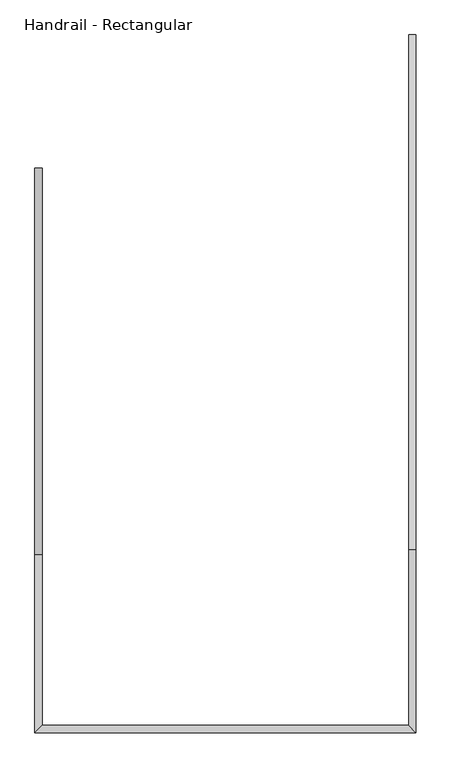
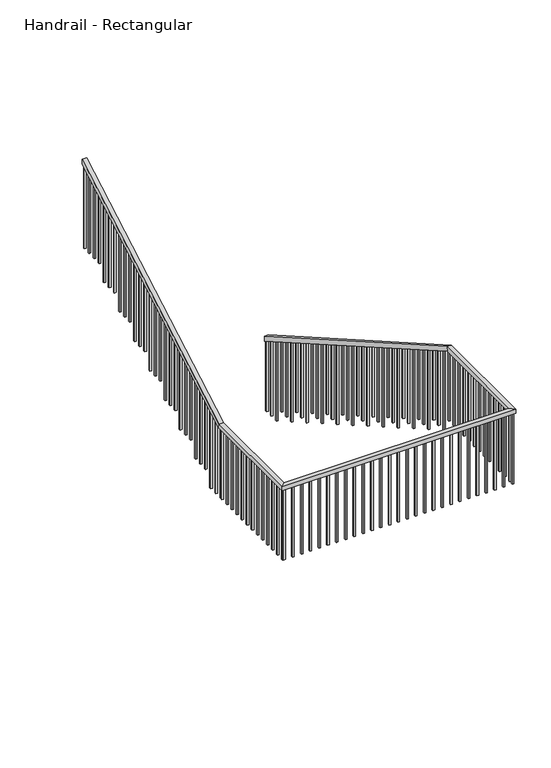
"""IFC4 building model written with IfcOpenShell, lengths in millimetres: railing geometry, Handrail - Rectangular."""

from ifc_helpers import new_model, si_unit, frame, origin, place, context, project, spatial, polyline, outline, extrude, faceted_brep, source, transform, mapped, element, save


def handrail_rectangular_c7adca0d(model_context):
    return source(origin(), model_context, "Body", "SolidModel", [
        faceted_brep([(-73282.7465, 13874.75, 13655.675), (-73282.7465, 13874.75, 13597.1285012), (-73333.5465, 13874.75, 13597.1285012), (-73333.5465, 13874.75, 13655.675), (-73282.7465, 10217.15, 15751.175), (-73282.7465, 10203.6288385, 15700.375), (-73333.5465, 10203.6288385, 15700.375), (-73333.5465, 10217.15, 15751.175), (-73282.7465, 8921.75, 15751.175), (-73282.7465, 8921.75, 15700.375), (-73333.5465, 8972.55, 15700.375), (-73333.5465, 8972.55, 15751.175), (-75987.8465, 8921.75, 15751.175), (-75987.8465, 8921.75, 15700.375), (-75937.0465, 8972.55, 15700.375), (-75937.0465, 8972.55, 15751.175), (-75987.8465, 10185.4, 15751.175), (-75987.8465, 10198.9211615, 15700.375), (-75937.0465, 10198.9211615, 15700.375), (-75937.0465, 10185.4, 15751.175), (-75987.8465, 12928.6, 17322.8), (-75937.0465, 12928.6, 17322.8), (-75937.0465, 12928.6, 17264.2535012), (-75987.8465, 12928.6, 17264.2535012)], [[[0, 1, 2, 3]], [[1, 0, 4, 5]], [[2, 1, 5, 6]], [[3, 2, 6, 7]], [[0, 3, 7, 4]], [[5, 4, 8, 9]], [[6, 5, 9, 10]], [[7, 6, 10, 11]], [[4, 7, 11, 8]], [[9, 8, 12, 13]], [[10, 9, 13, 14]], [[11, 10, 14, 15]], [[8, 11, 15, 12]], [[13, 12, 16, 17]], [[14, 13, 17, 18]], [[15, 14, 18, 19]], [[12, 15, 19, 16]], [[20, 21, 22, 23]], [[17, 16, 20, 23]], [[18, 17, 23, 22]], [[19, 18, 22, 21]], [[16, 19, 21, 20]]]),
        extrude(outline(polyline([(12836.525, 17211.5021992), (12836.525, 16233.775), (12817.475, 16233.775), (12817.475, 17200.5881367), (12836.525, 17211.5021992)])), frame((-75971.9715, 0.0, 0.0), z_axis=(1.0, 0.0, 0.0), x_axis=(0.0, 1.0, 0.0)), (0.0, 0.0, 1.0), 19.05),
        extrude(outline(polyline([(12734.925, 17153.2938658), (12734.925, 16233.775), (12715.875, 16233.775), (12715.875, 17142.3798033), (12734.925, 17153.2938658)])), frame((-75971.9715, 0.0, 0.0), z_axis=(1.0, 0.0, 0.0), x_axis=(0.0, 1.0, 0.0)), (0.0, 0.0, 1.0), 19.05),
        extrude(outline(polyline([(12633.325, 17095.0855325), (12633.325, 16233.775), (12614.275, 16233.775), (12614.275, 17084.17147), (12633.325, 17095.0855325)])), frame((-75971.9715, 0.0, 0.0), z_axis=(1.0, 0.0, 0.0), x_axis=(0.0, 1.0, 0.0)), (0.0, 0.0, 1.0), 19.05),
        extrude(outline(polyline([(12531.725, 17036.8771992), (12531.725, 16059.15), (12512.675, 16059.15), (12512.675, 17025.9631367), (12531.725, 17036.8771992)])), frame((-75971.9715, 0.0, 0.0), z_axis=(1.0, 0.0, 0.0), x_axis=(0.0, 1.0, 0.0)), (0.0, 0.0, 1.0), 19.05),
        extrude(outline(polyline([(12430.125, 16978.6688658), (12430.125, 16059.15), (12411.075, 16059.15), (12411.075, 16967.7548033), (12430.125, 16978.6688658)])), frame((-75971.9715, 0.0, 0.0), z_axis=(1.0, 0.0, 0.0), x_axis=(0.0, 1.0, 0.0)), (0.0, 0.0, 1.0), 19.05),
        extrude(outline(polyline([(12328.525, 16920.4605325), (12328.525, 16059.15), (12309.475, 16059.15), (12309.475, 16909.54647), (12328.525, 16920.4605325)])), frame((-75971.9715, 0.0, 0.0), z_axis=(1.0, 0.0, 0.0), x_axis=(0.0, 1.0, 0.0)), (0.0, 0.0, 1.0), 19.05),
        extrude(outline(polyline([(12226.925, 16862.2521992), (12226.925, 15884.525), (12207.875, 15884.525), (12207.875, 16851.3381367), (12226.925, 16862.2521992)])), frame((-75971.9715, 0.0, 0.0), z_axis=(1.0, 0.0, 0.0), x_axis=(0.0, 1.0, 0.0)), (0.0, 0.0, 1.0), 19.05),
        extrude(outline(polyline([(12125.325, 16804.0438658), (12125.325, 15884.525), (12106.275, 15884.525), (12106.275, 16793.1298033), (12125.325, 16804.0438658)])), frame((-75971.9715, 0.0, 0.0), z_axis=(1.0, 0.0, 0.0), x_axis=(0.0, 1.0, 0.0)), (0.0, 0.0, 1.0), 19.05),
        extrude(outline(polyline([(12023.725, 16745.8355325), (12023.725, 15884.525), (12004.675, 15884.525), (12004.675, 16734.92147), (12023.725, 16745.8355325)])), frame((-75971.9715, 0.0, 0.0), z_axis=(1.0, 0.0, 0.0), x_axis=(0.0, 1.0, 0.0)), (0.0, 0.0, 1.0), 19.05),
        extrude(outline(polyline([(11922.125, 16687.6271992), (11922.125, 15709.9), (11903.075, 15709.9), (11903.075, 16676.7131367), (11922.125, 16687.6271992)])), frame((-75971.9715, 0.0, 0.0), z_axis=(1.0, 0.0, 0.0), x_axis=(0.0, 1.0, 0.0)), (0.0, 0.0, 1.0), 19.05),
        extrude(outline(polyline([(11820.525, 16629.4188658), (11820.525, 15709.9), (11801.475, 15709.9), (11801.475, 16618.5048033), (11820.525, 16629.4188658)])), frame((-75971.9715, 0.0, 0.0), z_axis=(1.0, 0.0, 0.0), x_axis=(0.0, 1.0, 0.0)), (0.0, 0.0, 1.0), 19.05),
        extrude(outline(polyline([(11718.925, 16571.2105325), (11718.925, 15709.9), (11699.875, 15709.9), (11699.875, 16560.29647), (11718.925, 16571.2105325)])), frame((-75971.9715, 0.0, 0.0), z_axis=(1.0, 0.0, 0.0), x_axis=(0.0, 1.0, 0.0)), (0.0, 0.0, 1.0), 19.05),
        extrude(outline(polyline([(11617.325, 16513.0021992), (11617.325, 15535.275), (11598.275, 15535.275), (11598.275, 16502.0881367), (11617.325, 16513.0021992)])), frame((-75971.9715, 0.0, 0.0), z_axis=(1.0, 0.0, 0.0), x_axis=(0.0, 1.0, 0.0)), (0.0, 0.0, 1.0), 19.05),
        extrude(outline(polyline([(11515.725, 16454.7938658), (11515.725, 15535.275), (11496.675, 15535.275), (11496.675, 16443.8798033), (11515.725, 16454.7938658)])), frame((-75971.9715, 0.0, 0.0), z_axis=(1.0, 0.0, 0.0), x_axis=(0.0, 1.0, 0.0)), (0.0, 0.0, 1.0), 19.05),
        extrude(outline(polyline([(11414.125, 16396.5855325), (11414.125, 15535.275), (11395.075, 15535.275), (11395.075, 16385.67147), (11414.125, 16396.5855325)])), frame((-75971.9715, 0.0, 0.0), z_axis=(1.0, 0.0, 0.0), x_axis=(0.0, 1.0, 0.0)), (0.0, 0.0, 1.0), 19.05),
        extrude(outline(polyline([(11312.525, 16338.3771992), (11312.525, 15360.65), (11293.475, 15360.65), (11293.475, 16327.4631367), (11312.525, 16338.3771992)])), frame((-75971.9715, 0.0, 0.0), z_axis=(1.0, 0.0, 0.0), x_axis=(0.0, 1.0, 0.0)), (0.0, 0.0, 1.0), 19.05),
        extrude(outline(polyline([(11210.925, 16280.1688658), (11210.925, 15360.65), (11191.875, 15360.65), (11191.875, 16269.2548033), (11210.925, 16280.1688658)])), frame((-75971.9715, 0.0, 0.0), z_axis=(1.0, 0.0, 0.0), x_axis=(0.0, 1.0, 0.0)), (0.0, 0.0, 1.0), 19.05),
        extrude(outline(polyline([(11109.325, 16221.9605325), (11109.325, 15360.65), (11090.275, 15360.65), (11090.275, 16211.04647), (11109.325, 16221.9605325)])), frame((-75971.9715, 0.0, 0.0), z_axis=(1.0, 0.0, 0.0), x_axis=(0.0, 1.0, 0.0)), (0.0, 0.0, 1.0), 19.05),
        extrude(outline(polyline([(11007.725, 16163.7521992), (11007.725, 15186.025), (10988.675, 15186.025), (10988.675, 16152.8381367), (11007.725, 16163.7521992)])), frame((-75971.9715, 0.0, 0.0), z_axis=(1.0, 0.0, 0.0), x_axis=(0.0, 1.0, 0.0)), (0.0, 0.0, 1.0), 19.05),
        extrude(outline(polyline([(10906.125, 16105.5438658), (10906.125, 15186.025), (10887.075, 15186.025), (10887.075, 16094.6298033), (10906.125, 16105.5438658)])), frame((-75971.9715, 0.0, 0.0), z_axis=(1.0, 0.0, 0.0), x_axis=(0.0, 1.0, 0.0)), (0.0, 0.0, 1.0), 19.05),
        extrude(outline(polyline([(10804.525, 16047.3355325), (10804.525, 15186.025), (10785.475, 15186.025), (10785.475, 16036.42147), (10804.525, 16047.3355325)])), frame((-75971.9715, 0.0, 0.0), z_axis=(1.0, 0.0, 0.0), x_axis=(0.0, 1.0, 0.0)), (0.0, 0.0, 1.0), 19.05),
        extrude(outline(polyline([(10702.925, 15989.1271992), (10702.925, 15011.4), (10683.875, 15011.4), (10683.875, 15978.2131367), (10702.925, 15989.1271992)])), frame((-75971.9715, 0.0, 0.0), z_axis=(1.0, 0.0, 0.0), x_axis=(0.0, 1.0, 0.0)), (0.0, 0.0, 1.0), 19.05),
        extrude(outline(polyline([(10601.325, 15930.9188658), (10601.325, 15011.4), (10582.275, 15011.4), (10582.275, 15920.0048033), (10601.325, 15930.9188658)])), frame((-75971.9715, 0.0, 0.0), z_axis=(1.0, 0.0, 0.0), x_axis=(0.0, 1.0, 0.0)), (0.0, 0.0, 1.0), 19.05),
        extrude(outline(polyline([(10499.725, 15872.7105325), (10499.725, 15011.4), (10480.675, 15011.4), (10480.675, 15861.79647), (10499.725, 15872.7105325)])), frame((-75971.9715, 0.0, 0.0), z_axis=(1.0, 0.0, 0.0), x_axis=(0.0, 1.0, 0.0)), (0.0, 0.0, 1.0), 19.05),
        extrude(outline(polyline([(10398.125, 15814.5021992), (10398.125, 14836.775), (10379.075, 14836.775), (10379.075, 15803.5881367), (10398.125, 15814.5021992)])), frame((-75971.9715, 0.0, 0.0), z_axis=(1.0, 0.0, 0.0), x_axis=(0.0, 1.0, 0.0)), (0.0, 0.0, 1.0), 19.05),
        extrude(outline(polyline([(10296.525, 15756.2938658), (10296.525, 14836.775), (10277.475, 14836.775), (10277.475, 15745.3798033), (10296.525, 15756.2938658)])), frame((-75971.9715, 0.0, 0.0), z_axis=(1.0, 0.0, 0.0), x_axis=(0.0, 1.0, 0.0)), (0.0, 0.0, 1.0), 19.05),
        extrude(outline(polyline([(-75971.9715, 10156.825), (-75971.9715, 10175.875), (-75952.9215, 10175.875), (-75952.9215, 10156.825), (-75971.9715, 10156.825)])), frame((0.0, 0.0, 14836.775), z_axis=(0.0, 0.0, 1.0), x_axis=(1.0, 0.0, 0.0)), (0.0, 0.0, 1.0), 863.6),
        extrude(outline(polyline([(-75971.9715, 10055.225), (-75971.9715, 10074.275), (-75952.9215, 10074.275), (-75952.9215, 10055.225), (-75971.9715, 10055.225)])), frame((0.0, 0.0, 14836.775), z_axis=(0.0, 0.0, 1.0), x_axis=(1.0, 0.0, 0.0)), (0.0, 0.0, 1.0), 863.6),
        extrude(outline(polyline([(-75971.9715, 9953.625), (-75971.9715, 9972.675), (-75952.9215, 9972.675), (-75952.9215, 9953.625), (-75971.9715, 9953.625)])), frame((0.0, 0.0, 14836.775), z_axis=(0.0, 0.0, 1.0), x_axis=(1.0, 0.0, 0.0)), (0.0, 0.0, 1.0), 863.6),
        extrude(outline(polyline([(-75971.9715, 9852.025), (-75971.9715, 9871.075), (-75952.9215, 9871.075), (-75952.9215, 9852.025), (-75971.9715, 9852.025)])), frame((0.0, 0.0, 14836.775), z_axis=(0.0, 0.0, 1.0), x_axis=(1.0, 0.0, 0.0)), (0.0, 0.0, 1.0), 863.6),
        extrude(outline(polyline([(-75971.9715, 9750.425), (-75971.9715, 9769.475), (-75952.9215, 9769.475), (-75952.9215, 9750.425), (-75971.9715, 9750.425)])), frame((0.0, 0.0, 14836.775), z_axis=(0.0, 0.0, 1.0), x_axis=(1.0, 0.0, 0.0)), (0.0, 0.0, 1.0), 863.6),
        extrude(outline(polyline([(-75971.9715, 9648.825), (-75971.9715, 9667.875), (-75952.9215, 9667.875), (-75952.9215, 9648.825), (-75971.9715, 9648.825)])), frame((0.0, 0.0, 14836.775), z_axis=(0.0, 0.0, 1.0), x_axis=(1.0, 0.0, 0.0)), (0.0, 0.0, 1.0), 863.6),
        extrude(outline(polyline([(-75971.9715, 9547.225), (-75971.9715, 9566.275), (-75952.9215, 9566.275), (-75952.9215, 9547.225), (-75971.9715, 9547.225)])), frame((0.0, 0.0, 14836.775), z_axis=(0.0, 0.0, 1.0), x_axis=(1.0, 0.0, 0.0)), (0.0, 0.0, 1.0), 863.6),
        extrude(outline(polyline([(-75971.9715, 9445.625), (-75971.9715, 9464.675), (-75952.9215, 9464.675), (-75952.9215, 9445.625), (-75971.9715, 9445.625)])), frame((0.0, 0.0, 14836.775), z_axis=(0.0, 0.0, 1.0), x_axis=(1.0, 0.0, 0.0)), (0.0, 0.0, 1.0), 863.6),
        extrude(outline(polyline([(-75971.9715, 9344.025), (-75971.9715, 9363.075), (-75952.9215, 9363.075), (-75952.9215, 9344.025), (-75971.9715, 9344.025)])), frame((0.0, 0.0, 14836.775), z_axis=(0.0, 0.0, 1.0), x_axis=(1.0, 0.0, 0.0)), (0.0, 0.0, 1.0), 863.6),
        extrude(outline(polyline([(-75971.9715, 9242.425), (-75971.9715, 9261.475), (-75952.9215, 9261.475), (-75952.9215, 9242.425), (-75971.9715, 9242.425)])), frame((0.0, 0.0, 14836.775), z_axis=(0.0, 0.0, 1.0), x_axis=(1.0, 0.0, 0.0)), (0.0, 0.0, 1.0), 863.6),
        extrude(outline(polyline([(-75971.9715, 9140.825), (-75971.9715, 9159.875), (-75952.9215, 9159.875), (-75952.9215, 9140.825), (-75971.9715, 9140.825)])), frame((0.0, 0.0, 14836.775), z_axis=(0.0, 0.0, 1.0), x_axis=(1.0, 0.0, 0.0)), (0.0, 0.0, 1.0), 863.6),
        extrude(outline(polyline([(-75971.9715, 9039.225), (-75971.9715, 9058.275), (-75952.9215, 9058.275), (-75952.9215, 9039.225), (-75971.9715, 9039.225)])), frame((0.0, 0.0, 14836.775), z_axis=(0.0, 0.0, 1.0), x_axis=(1.0, 0.0, 0.0)), (0.0, 0.0, 1.0), 863.6),
        extrude(outline(polyline([(-75940.2215, 8937.625), (-75959.2715, 8937.625), (-75959.2715, 8956.675), (-75940.2215, 8956.675), (-75940.2215, 8937.625)])), frame((0.0, 0.0, 14836.775), z_axis=(0.0, 0.0, 1.0), x_axis=(1.0, 0.0, 0.0)), (0.0, 0.0, 1.0), 863.6),
        extrude(outline(polyline([(-75838.6215, 8937.625), (-75857.6715, 8937.625), (-75857.6715, 8956.675), (-75838.6215, 8956.675), (-75838.6215, 8937.625)])), frame((0.0, 0.0, 14836.775), z_axis=(0.0, 0.0, 1.0), x_axis=(1.0, 0.0, 0.0)), (0.0, 0.0, 1.0), 863.6),
        extrude(outline(polyline([(-75737.0215, 8937.625), (-75756.0715, 8937.625), (-75756.0715, 8956.675), (-75737.0215, 8956.675), (-75737.0215, 8937.625)])), frame((0.0, 0.0, 14836.775), z_axis=(0.0, 0.0, 1.0), x_axis=(1.0, 0.0, 0.0)), (0.0, 0.0, 1.0), 863.6),
        extrude(outline(polyline([(-75635.4215, 8937.625), (-75654.4715, 8937.625), (-75654.4715, 8956.675), (-75635.4215, 8956.675), (-75635.4215, 8937.625)])), frame((0.0, 0.0, 14836.775), z_axis=(0.0, 0.0, 1.0), x_axis=(1.0, 0.0, 0.0)), (0.0, 0.0, 1.0), 863.6),
        extrude(outline(polyline([(-75533.8215, 8937.625), (-75552.8715, 8937.625), (-75552.8715, 8956.675), (-75533.8215, 8956.675), (-75533.8215, 8937.625)])), frame((0.0, 0.0, 14836.775), z_axis=(0.0, 0.0, 1.0), x_axis=(1.0, 0.0, 0.0)), (0.0, 0.0, 1.0), 863.6),
        extrude(outline(polyline([(-75432.2215, 8937.625), (-75451.2715, 8937.625), (-75451.2715, 8956.675), (-75432.2215, 8956.675), (-75432.2215, 8937.625)])), frame((0.0, 0.0, 14836.775), z_axis=(0.0, 0.0, 1.0), x_axis=(1.0, 0.0, 0.0)), (0.0, 0.0, 1.0), 863.6),
        extrude(outline(polyline([(-75330.6215, 8937.625), (-75349.6715, 8937.625), (-75349.6715, 8956.675), (-75330.6215, 8956.675), (-75330.6215, 8937.625)])), frame((0.0, 0.0, 14836.775), z_axis=(0.0, 0.0, 1.0), x_axis=(1.0, 0.0, 0.0)), (0.0, 0.0, 1.0), 863.6),
        extrude(outline(polyline([(-75229.0215, 8937.625), (-75248.0715, 8937.625), (-75248.0715, 8956.675), (-75229.0215, 8956.675), (-75229.0215, 8937.625)])), frame((0.0, 0.0, 14836.775), z_axis=(0.0, 0.0, 1.0), x_axis=(1.0, 0.0, 0.0)), (0.0, 0.0, 1.0), 863.6),
        extrude(outline(polyline([(-75127.4215, 8937.625), (-75146.4715, 8937.625), (-75146.4715, 8956.675), (-75127.4215, 8956.675), (-75127.4215, 8937.625)])), frame((0.0, 0.0, 14836.775), z_axis=(0.0, 0.0, 1.0), x_axis=(1.0, 0.0, 0.0)), (0.0, 0.0, 1.0), 863.6),
        extrude(outline(polyline([(-75025.8215, 8937.625), (-75044.8715, 8937.625), (-75044.8715, 8956.675), (-75025.8215, 8956.675), (-75025.8215, 8937.625)])), frame((0.0, 0.0, 14836.775), z_axis=(0.0, 0.0, 1.0), x_axis=(1.0, 0.0, 0.0)), (0.0, 0.0, 1.0), 863.6),
        extrude(outline(polyline([(-74924.2215, 8937.625), (-74943.2715, 8937.625), (-74943.2715, 8956.675), (-74924.2215, 8956.675), (-74924.2215, 8937.625)])), frame((0.0, 0.0, 14836.775), z_axis=(0.0, 0.0, 1.0), x_axis=(1.0, 0.0, 0.0)), (0.0, 0.0, 1.0), 863.6),
        extrude(outline(polyline([(-74822.6215, 8937.625), (-74841.6715, 8937.625), (-74841.6715, 8956.675), (-74822.6215, 8956.675), (-74822.6215, 8937.625)])), frame((0.0, 0.0, 14836.775), z_axis=(0.0, 0.0, 1.0), x_axis=(1.0, 0.0, 0.0)), (0.0, 0.0, 1.0), 863.6),
        extrude(outline(polyline([(-74721.0215, 8937.625), (-74740.0715, 8937.625), (-74740.0715, 8956.675), (-74721.0215, 8956.675), (-74721.0215, 8937.625)])), frame((0.0, 0.0, 14836.775), z_axis=(0.0, 0.0, 1.0), x_axis=(1.0, 0.0, 0.0)), (0.0, 0.0, 1.0), 863.6),
        extrude(outline(polyline([(-74619.4215, 8937.625), (-74638.4715, 8937.625), (-74638.4715, 8956.675), (-74619.4215, 8956.675), (-74619.4215, 8937.625)])), frame((0.0, 0.0, 14836.775), z_axis=(0.0, 0.0, 1.0), x_axis=(1.0, 0.0, 0.0)), (0.0, 0.0, 1.0), 863.6),
        extrude(outline(polyline([(-74517.8215, 8937.625), (-74536.8715, 8937.625), (-74536.8715, 8956.675), (-74517.8215, 8956.675), (-74517.8215, 8937.625)])), frame((0.0, 0.0, 14836.775), z_axis=(0.0, 0.0, 1.0), x_axis=(1.0, 0.0, 0.0)), (0.0, 0.0, 1.0), 863.6),
        extrude(outline(polyline([(-74416.2215, 8937.625), (-74435.2715, 8937.625), (-74435.2715, 8956.675), (-74416.2215, 8956.675), (-74416.2215, 8937.625)])), frame((0.0, 0.0, 14836.775), z_axis=(0.0, 0.0, 1.0), x_axis=(1.0, 0.0, 0.0)), (0.0, 0.0, 1.0), 863.6),
        extrude(outline(polyline([(-74314.6215, 8937.625), (-74333.6715, 8937.625), (-74333.6715, 8956.675), (-74314.6215, 8956.675), (-74314.6215, 8937.625)])), frame((0.0, 0.0, 14836.775), z_axis=(0.0, 0.0, 1.0), x_axis=(1.0, 0.0, 0.0)), (0.0, 0.0, 1.0), 863.6),
        extrude(outline(polyline([(-74213.0215, 8937.625), (-74232.0715, 8937.625), (-74232.0715, 8956.675), (-74213.0215, 8956.675), (-74213.0215, 8937.625)])), frame((0.0, 0.0, 14836.775), z_axis=(0.0, 0.0, 1.0), x_axis=(1.0, 0.0, 0.0)), (0.0, 0.0, 1.0), 863.6),
        extrude(outline(polyline([(-74111.4215, 8937.625), (-74130.4715, 8937.625), (-74130.4715, 8956.675), (-74111.4215, 8956.675), (-74111.4215, 8937.625)])), frame((0.0, 0.0, 14836.775), z_axis=(0.0, 0.0, 1.0), x_axis=(1.0, 0.0, 0.0)), (0.0, 0.0, 1.0), 863.6),
        extrude(outline(polyline([(-74009.8215, 8937.625), (-74028.8715, 8937.625), (-74028.8715, 8956.675), (-74009.8215, 8956.675), (-74009.8215, 8937.625)])), frame((0.0, 0.0, 14836.775), z_axis=(0.0, 0.0, 1.0), x_axis=(1.0, 0.0, 0.0)), (0.0, 0.0, 1.0), 863.6),
        extrude(outline(polyline([(-73908.2215, 8937.625), (-73927.2715, 8937.625), (-73927.2715, 8956.675), (-73908.2215, 8956.675), (-73908.2215, 8937.625)])), frame((0.0, 0.0, 14836.775), z_axis=(0.0, 0.0, 1.0), x_axis=(1.0, 0.0, 0.0)), (0.0, 0.0, 1.0), 863.6),
        extrude(outline(polyline([(-73806.6215, 8937.625), (-73825.6715, 8937.625), (-73825.6715, 8956.675), (-73806.6215, 8956.675), (-73806.6215, 8937.625)])), frame((0.0, 0.0, 14836.775), z_axis=(0.0, 0.0, 1.0), x_axis=(1.0, 0.0, 0.0)), (0.0, 0.0, 1.0), 863.6),
        extrude(outline(polyline([(-73705.0215, 8937.625), (-73724.0715, 8937.625), (-73724.0715, 8956.675), (-73705.0215, 8956.675), (-73705.0215, 8937.625)])), frame((0.0, 0.0, 14836.775), z_axis=(0.0, 0.0, 1.0), x_axis=(1.0, 0.0, 0.0)), (0.0, 0.0, 1.0), 863.6),
        extrude(outline(polyline([(-73603.4215, 8937.625), (-73622.4715, 8937.625), (-73622.4715, 8956.675), (-73603.4215, 8956.675), (-73603.4215, 8937.625)])), frame((0.0, 0.0, 14836.775), z_axis=(0.0, 0.0, 1.0), x_axis=(1.0, 0.0, 0.0)), (0.0, 0.0, 1.0), 863.6),
        extrude(outline(polyline([(-73501.8215, 8937.625), (-73520.8715, 8937.625), (-73520.8715, 8956.675), (-73501.8215, 8956.675), (-73501.8215, 8937.625)])), frame((0.0, 0.0, 14836.775), z_axis=(0.0, 0.0, 1.0), x_axis=(1.0, 0.0, 0.0)), (0.0, 0.0, 1.0), 863.6),
        extrude(outline(polyline([(-73400.2215, 8937.625), (-73419.2715, 8937.625), (-73419.2715, 8956.675), (-73400.2215, 8956.675), (-73400.2215, 8937.625)])), frame((0.0, 0.0, 14836.775), z_axis=(0.0, 0.0, 1.0), x_axis=(1.0, 0.0, 0.0)), (0.0, 0.0, 1.0), 863.6),
        extrude(outline(polyline([(-73298.6215, 9007.475), (-73298.6215, 8988.425), (-73317.6715, 8988.425), (-73317.6715, 9007.475), (-73298.6215, 9007.475)])), frame((0.0, 0.0, 14836.775), z_axis=(0.0, 0.0, 1.0), x_axis=(1.0, 0.0, 0.0)), (0.0, 0.0, 1.0), 863.6),
        extrude(outline(polyline([(-73298.6215, 9109.075), (-73298.6215, 9090.025), (-73317.6715, 9090.025), (-73317.6715, 9109.075), (-73298.6215, 9109.075)])), frame((0.0, 0.0, 14836.775), z_axis=(0.0, 0.0, 1.0), x_axis=(1.0, 0.0, 0.0)), (0.0, 0.0, 1.0), 863.6),
        extrude(outline(polyline([(-73298.6215, 9210.675), (-73298.6215, 9191.625), (-73317.6715, 9191.625), (-73317.6715, 9210.675), (-73298.6215, 9210.675)])), frame((0.0, 0.0, 14836.775), z_axis=(0.0, 0.0, 1.0), x_axis=(1.0, 0.0, 0.0)), (0.0, 0.0, 1.0), 863.6),
        extrude(outline(polyline([(-73298.6215, 9312.275), (-73298.6215, 9293.225), (-73317.6715, 9293.225), (-73317.6715, 9312.275), (-73298.6215, 9312.275)])), frame((0.0, 0.0, 14836.775), z_axis=(0.0, 0.0, 1.0), x_axis=(1.0, 0.0, 0.0)), (0.0, 0.0, 1.0), 863.6),
        extrude(outline(polyline([(-73298.6215, 9413.875), (-73298.6215, 9394.825), (-73317.6715, 9394.825), (-73317.6715, 9413.875), (-73298.6215, 9413.875)])), frame((0.0, 0.0, 14836.775), z_axis=(0.0, 0.0, 1.0), x_axis=(1.0, 0.0, 0.0)), (0.0, 0.0, 1.0), 863.6),
        extrude(outline(polyline([(-73298.6215, 9515.475), (-73298.6215, 9496.425), (-73317.6715, 9496.425), (-73317.6715, 9515.475), (-73298.6215, 9515.475)])), frame((0.0, 0.0, 14836.775), z_axis=(0.0, 0.0, 1.0), x_axis=(1.0, 0.0, 0.0)), (0.0, 0.0, 1.0), 863.6),
        extrude(outline(polyline([(-73298.6215, 9617.075), (-73298.6215, 9598.025), (-73317.6715, 9598.025), (-73317.6715, 9617.075), (-73298.6215, 9617.075)])), frame((0.0, 0.0, 14836.775), z_axis=(0.0, 0.0, 1.0), x_axis=(1.0, 0.0, 0.0)), (0.0, 0.0, 1.0), 863.6),
        extrude(outline(polyline([(-73298.6215, 9718.675), (-73298.6215, 9699.625), (-73317.6715, 9699.625), (-73317.6715, 9718.675), (-73298.6215, 9718.675)])), frame((0.0, 0.0, 14836.775), z_axis=(0.0, 0.0, 1.0), x_axis=(1.0, 0.0, 0.0)), (0.0, 0.0, 1.0), 863.6),
        extrude(outline(polyline([(-73298.6215, 9820.275), (-73298.6215, 9801.225), (-73317.6715, 9801.225), (-73317.6715, 9820.275), (-73298.6215, 9820.275)])), frame((0.0, 0.0, 14836.775), z_axis=(0.0, 0.0, 1.0), x_axis=(1.0, 0.0, 0.0)), (0.0, 0.0, 1.0), 863.6),
        extrude(outline(polyline([(-73298.6215, 9921.875), (-73298.6215, 9902.825), (-73317.6715, 9902.825), (-73317.6715, 9921.875), (-73298.6215, 9921.875)])), frame((0.0, 0.0, 14836.775), z_axis=(0.0, 0.0, 1.0), x_axis=(1.0, 0.0, 0.0)), (0.0, 0.0, 1.0), 863.6),
        extrude(outline(polyline([(-73298.6215, 10023.475), (-73298.6215, 10004.425), (-73317.6715, 10004.425), (-73317.6715, 10023.475), (-73298.6215, 10023.475)])), frame((0.0, 0.0, 14836.775), z_axis=(0.0, 0.0, 1.0), x_axis=(1.0, 0.0, 0.0)), (0.0, 0.0, 1.0), 863.6),
        extrude(outline(polyline([(-73298.6215, 10125.075), (-73298.6215, 10106.025), (-73317.6715, 10106.025), (-73317.6715, 10125.075), (-73298.6215, 10125.075)])), frame((0.0, 0.0, 14836.775), z_axis=(0.0, 0.0, 1.0), x_axis=(1.0, 0.0, 0.0)), (0.0, 0.0, 1.0), 863.6),
        extrude(outline(polyline([(10328.275, 15628.9631367), (10328.275, 14662.15), (10309.225, 14662.15), (10309.225, 15639.8771992), (10328.275, 15628.9631367)])), frame((-73317.6715, 0.0, 0.0), z_axis=(1.0, 0.0, 0.0), x_axis=(0.0, 1.0, 0.0)), (0.0, 0.0, 1.0), 19.05),
        extrude(outline(polyline([(10429.875, 15570.7548033), (10429.875, 14662.15), (10410.825, 14662.15), (10410.825, 15581.6688658), (10429.875, 15570.7548033)])), frame((-73317.6715, 0.0, 0.0), z_axis=(1.0, 0.0, 0.0), x_axis=(0.0, 1.0, 0.0)), (0.0, 0.0, 1.0), 19.05),
        extrude(outline(polyline([(10531.475, 15512.54647), (10531.475, 14662.15), (10512.425, 14662.15), (10512.425, 15523.4605325), (10531.475, 15512.54647)])), frame((-73317.6715, 0.0, 0.0), z_axis=(1.0, 0.0, 0.0), x_axis=(0.0, 1.0, 0.0)), (0.0, 0.0, 1.0), 19.05),
        extrude(outline(polyline([(10633.075, 15454.3381367), (10633.075, 14487.525), (10614.025, 14487.525), (10614.025, 15465.2521992), (10633.075, 15454.3381367)])), frame((-73317.6715, 0.0, 0.0), z_axis=(1.0, 0.0, 0.0), x_axis=(0.0, 1.0, 0.0)), (0.0, 0.0, 1.0), 19.05),
        extrude(outline(polyline([(10734.675, 15396.1298033), (10734.675, 14487.525), (10715.625, 14487.525), (10715.625, 15407.0438658), (10734.675, 15396.1298033)])), frame((-73317.6715, 0.0, 0.0), z_axis=(1.0, 0.0, 0.0), x_axis=(0.0, 1.0, 0.0)), (0.0, 0.0, 1.0), 19.05),
        extrude(outline(polyline([(10836.275, 15337.92147), (10836.275, 14487.525), (10817.225, 14487.525), (10817.225, 15348.8355325), (10836.275, 15337.92147)])), frame((-73317.6715, 0.0, 0.0), z_axis=(1.0, 0.0, 0.0), x_axis=(0.0, 1.0, 0.0)), (0.0, 0.0, 1.0), 19.05),
        extrude(outline(polyline([(10937.875, 15279.7131367), (10937.875, 14312.9), (10918.825, 14312.9), (10918.825, 15290.6271992), (10937.875, 15279.7131367)])), frame((-73317.6715, 0.0, 0.0), z_axis=(1.0, 0.0, 0.0), x_axis=(0.0, 1.0, 0.0)), (0.0, 0.0, 1.0), 19.05),
        extrude(outline(polyline([(11039.475, 15221.5048033), (11039.475, 14312.9), (11020.425, 14312.9), (11020.425, 15232.4188658), (11039.475, 15221.5048033)])), frame((-73317.6715, 0.0, 0.0), z_axis=(1.0, 0.0, 0.0), x_axis=(0.0, 1.0, 0.0)), (0.0, 0.0, 1.0), 19.05),
        extrude(outline(polyline([(11141.075, 15163.29647), (11141.075, 14312.9), (11122.025, 14312.9), (11122.025, 15174.2105325), (11141.075, 15163.29647)])), frame((-73317.6715, 0.0, 0.0), z_axis=(1.0, 0.0, 0.0), x_axis=(0.0, 1.0, 0.0)), (0.0, 0.0, 1.0), 19.05),
        extrude(outline(polyline([(11242.675, 15105.0881367), (11242.675, 14138.275), (11223.625, 14138.275), (11223.625, 15116.0021992), (11242.675, 15105.0881367)])), frame((-73317.6715, 0.0, 0.0), z_axis=(1.0, 0.0, 0.0), x_axis=(0.0, 1.0, 0.0)), (0.0, 0.0, 1.0), 19.05),
        extrude(outline(polyline([(11344.275, 15046.8798033), (11344.275, 14138.275), (11325.225, 14138.275), (11325.225, 15057.7938658), (11344.275, 15046.8798033)])), frame((-73317.6715, 0.0, 0.0), z_axis=(1.0, 0.0, 0.0), x_axis=(0.0, 1.0, 0.0)), (0.0, 0.0, 1.0), 19.05),
        extrude(outline(polyline([(11445.875, 14988.67147), (11445.875, 14138.275), (11426.825, 14138.275), (11426.825, 14999.5855325), (11445.875, 14988.67147)])), frame((-73317.6715, 0.0, 0.0), z_axis=(1.0, 0.0, 0.0), x_axis=(0.0, 1.0, 0.0)), (0.0, 0.0, 1.0), 19.05),
        extrude(outline(polyline([(11547.475, 14930.4631367), (11547.475, 13963.65), (11528.425, 13963.65), (11528.425, 14941.3771992), (11547.475, 14930.4631367)])), frame((-73317.6715, 0.0, 0.0), z_axis=(1.0, 0.0, 0.0), x_axis=(0.0, 1.0, 0.0)), (0.0, 0.0, 1.0), 19.05),
        extrude(outline(polyline([(11649.075, 14872.2548033), (11649.075, 13963.65), (11630.025, 13963.65), (11630.025, 14883.1688658), (11649.075, 14872.2548033)])), frame((-73317.6715, 0.0, 0.0), z_axis=(1.0, 0.0, 0.0), x_axis=(0.0, 1.0, 0.0)), (0.0, 0.0, 1.0), 19.05),
        extrude(outline(polyline([(11750.675, 14814.04647), (11750.675, 13963.65), (11731.625, 13963.65), (11731.625, 14824.9605325), (11750.675, 14814.04647)])), frame((-73317.6715, 0.0, 0.0), z_axis=(1.0, 0.0, 0.0), x_axis=(0.0, 1.0, 0.0)), (0.0, 0.0, 1.0), 19.05),
        extrude(outline(polyline([(11852.275, 14755.8381367), (11852.275, 13789.025), (11833.225, 13789.025), (11833.225, 14766.7521992), (11852.275, 14755.8381367)])), frame((-73317.6715, 0.0, 0.0), z_axis=(1.0, 0.0, 0.0), x_axis=(0.0, 1.0, 0.0)), (0.0, 0.0, 1.0), 19.05),
        extrude(outline(polyline([(11953.875, 14697.6298033), (11953.875, 13789.025), (11934.825, 13789.025), (11934.825, 14708.5438658), (11953.875, 14697.6298033)])), frame((-73317.6715, 0.0, 0.0), z_axis=(1.0, 0.0, 0.0), x_axis=(0.0, 1.0, 0.0)), (0.0, 0.0, 1.0), 19.05),
        extrude(outline(polyline([(12055.475, 14639.42147), (12055.475, 13789.025), (12036.425, 13789.025), (12036.425, 14650.3355325), (12055.475, 14639.42147)])), frame((-73317.6715, 0.0, 0.0), z_axis=(1.0, 0.0, 0.0), x_axis=(0.0, 1.0, 0.0)), (0.0, 0.0, 1.0), 19.05),
        extrude(outline(polyline([(12157.075, 14581.2131367), (12157.075, 13614.4), (12138.025, 13614.4), (12138.025, 14592.1271992), (12157.075, 14581.2131367)])), frame((-73317.6715, 0.0, 0.0), z_axis=(1.0, 0.0, 0.0), x_axis=(0.0, 1.0, 0.0)), (0.0, 0.0, 1.0), 19.05),
        extrude(outline(polyline([(12258.675, 14523.0048033), (12258.675, 13614.4), (12239.625, 13614.4), (12239.625, 14533.9188658), (12258.675, 14523.0048033)])), frame((-73317.6715, 0.0, 0.0), z_axis=(1.0, 0.0, 0.0), x_axis=(0.0, 1.0, 0.0)), (0.0, 0.0, 1.0), 19.05),
        extrude(outline(polyline([(12360.275, 14464.79647), (12360.275, 13614.4), (12341.225, 13614.4), (12341.225, 14475.7105325), (12360.275, 14464.79647)])), frame((-73317.6715, 0.0, 0.0), z_axis=(1.0, 0.0, 0.0), x_axis=(0.0, 1.0, 0.0)), (0.0, 0.0, 1.0), 19.05),
        extrude(outline(polyline([(12461.875, 14406.5881367), (12461.875, 13439.775), (12442.825, 13439.775), (12442.825, 14417.5021992), (12461.875, 14406.5881367)])), frame((-73317.6715, 0.0, 0.0), z_axis=(1.0, 0.0, 0.0), x_axis=(0.0, 1.0, 0.0)), (0.0, 0.0, 1.0), 19.05),
        extrude(outline(polyline([(12563.475, 14348.3798033), (12563.475, 13439.775), (12544.425, 13439.775), (12544.425, 14359.2938658), (12563.475, 14348.3798033)])), frame((-73317.6715, 0.0, 0.0), z_axis=(1.0, 0.0, 0.0), x_axis=(0.0, 1.0, 0.0)), (0.0, 0.0, 1.0), 19.05),
        extrude(outline(polyline([(12665.075, 14290.17147), (12665.075, 13439.775), (12646.025, 13439.775), (12646.025, 14301.0855325), (12665.075, 14290.17147)])), frame((-73317.6715, 0.0, 0.0), z_axis=(1.0, 0.0, 0.0), x_axis=(0.0, 1.0, 0.0)), (0.0, 0.0, 1.0), 19.05),
        extrude(outline(polyline([(12766.675, 14231.9631367), (12766.675, 13265.15), (12747.625, 13265.15), (12747.625, 14242.8771992), (12766.675, 14231.9631367)])), frame((-73317.6715, 0.0, 0.0), z_axis=(1.0, 0.0, 0.0), x_axis=(0.0, 1.0, 0.0)), (0.0, 0.0, 1.0), 19.05),
        extrude(outline(polyline([(12868.275, 14173.7548033), (12868.275, 13265.15), (12849.225, 13265.15), (12849.225, 14184.6688658), (12868.275, 14173.7548033)])), frame((-73317.6715, 0.0, 0.0), z_axis=(1.0, 0.0, 0.0), x_axis=(0.0, 1.0, 0.0)), (0.0, 0.0, 1.0), 19.05),
        extrude(outline(polyline([(12969.875, 14115.54647), (12969.875, 13265.15), (12950.825, 13265.15), (12950.825, 14126.4605325), (12969.875, 14115.54647)])), frame((-73317.6715, 0.0, 0.0), z_axis=(1.0, 0.0, 0.0), x_axis=(0.0, 1.0, 0.0)), (0.0, 0.0, 1.0), 19.05),
        extrude(outline(polyline([(13071.475, 14057.3381367), (13071.475, 13090.525), (13052.425, 13090.525), (13052.425, 14068.2521992), (13071.475, 14057.3381367)])), frame((-73317.6715, 0.0, 0.0), z_axis=(1.0, 0.0, 0.0), x_axis=(0.0, 1.0, 0.0)), (0.0, 0.0, 1.0), 19.05),
        extrude(outline(polyline([(13173.075, 13999.1298033), (13173.075, 13090.525), (13154.025, 13090.525), (13154.025, 14010.0438658), (13173.075, 13999.1298033)])), frame((-73317.6715, 0.0, 0.0), z_axis=(1.0, 0.0, 0.0), x_axis=(0.0, 1.0, 0.0)), (0.0, 0.0, 1.0), 19.05),
        extrude(outline(polyline([(13274.675, 13940.92147), (13274.675, 13090.525), (13255.625, 13090.525), (13255.625, 13951.8355325), (13274.675, 13940.92147)])), frame((-73317.6715, 0.0, 0.0), z_axis=(1.0, 0.0, 0.0), x_axis=(0.0, 1.0, 0.0)), (0.0, 0.0, 1.0), 19.05),
        extrude(outline(polyline([(13376.275, 13882.7131367), (13376.275, 12915.9), (13357.225, 12915.9), (13357.225, 13893.6271992), (13376.275, 13882.7131367)])), frame((-73317.6715, 0.0, 0.0), z_axis=(1.0, 0.0, 0.0), x_axis=(0.0, 1.0, 0.0)), (0.0, 0.0, 1.0), 19.05),
        extrude(outline(polyline([(13477.875, 13824.5048033), (13477.875, 12915.9), (13458.825, 12915.9), (13458.825, 13835.4188658), (13477.875, 13824.5048033)])), frame((-73317.6715, 0.0, 0.0), z_axis=(1.0, 0.0, 0.0), x_axis=(0.0, 1.0, 0.0)), (0.0, 0.0, 1.0), 19.05),
        extrude(outline(polyline([(13579.475, 13766.29647), (13579.475, 12915.9), (13560.425, 12915.9), (13560.425, 13777.2105325), (13579.475, 13766.29647)])), frame((-73317.6715, 0.0, 0.0), z_axis=(1.0, 0.0, 0.0), x_axis=(0.0, 1.0, 0.0)), (0.0, 0.0, 1.0), 19.05),
        extrude(outline(polyline([(13681.075, 13708.0881367), (13681.075, 12741.275), (13662.025, 12741.275), (13662.025, 13719.0021992), (13681.075, 13708.0881367)])), frame((-73317.6715, 0.0, 0.0), z_axis=(1.0, 0.0, 0.0), x_axis=(0.0, 1.0, 0.0)), (0.0, 0.0, 1.0), 19.05),
        extrude(outline(polyline([(13782.675, 13649.8798033), (13782.675, 12741.275), (13763.625, 12741.275), (13763.625, 13660.7938658), (13782.675, 13649.8798033)])), frame((-73317.6715, 0.0, 0.0), z_axis=(1.0, 0.0, 0.0), x_axis=(0.0, 1.0, 0.0)), (0.0, 0.0, 1.0), 19.05),
        extrude(outline(polyline([(-75971.9715, 10175.875), (-75971.9715, 10194.925), (-75952.9215, 10194.925), (-75952.9215, 10175.875), (-75971.9715, 10175.875)])), frame((0.0, 0.0, 14836.775), z_axis=(0.0, 0.0, 1.0), x_axis=(1.0, 0.0, 0.0)), (0.0, 0.0, 1.0), 863.6),
        extrude(outline(polyline([(-75952.9215, 8937.625), (-75971.9715, 8937.625), (-75971.9715, 8956.675), (-75952.9215, 8956.675), (-75952.9215, 8937.625)])), frame((0.0, 0.0, 14836.775), z_axis=(0.0, 0.0, 1.0), x_axis=(1.0, 0.0, 0.0)), (0.0, 0.0, 1.0), 863.6),
        extrude(outline(polyline([(-73298.6215, 8956.675), (-73298.6215, 8937.625), (-73317.6715, 8937.625), (-73317.6715, 8956.675), (-73298.6215, 8956.675)])), frame((0.0, 0.0, 14836.775), z_axis=(0.0, 0.0, 1.0), x_axis=(1.0, 0.0, 0.0)), (0.0, 0.0, 1.0), 863.6),
        extrude(outline(polyline([(-73298.6215, 10226.675), (-73298.6215, 10207.625), (-73317.6715, 10207.625), (-73317.6715, 10226.675), (-73298.6215, 10226.675)])), frame((0.0, 0.0, 14836.775), z_axis=(0.0, 0.0, 1.0), x_axis=(1.0, 0.0, 0.0)), (0.0, 0.0, 1.0), 863.6),
        extrude(outline(polyline([(12928.6, 17264.2535012), (12928.6, 16233.775), (12909.55, 16233.775), (12909.55, 17253.3394387), (12928.6, 17264.2535012)])), frame((-75971.9715, 0.0, 0.0), z_axis=(1.0, 0.0, 0.0), x_axis=(0.0, 1.0, 0.0)), (0.0, 0.0, 1.0), 19.05),
        extrude(outline(polyline([(13874.75, 13597.1285012), (13874.75, 12741.275), (13855.7, 12741.275), (13855.7, 13608.0425637), (13874.75, 13597.1285012)])), frame((-73317.6715, 0.0, 0.0), z_axis=(1.0, 0.0, 0.0), x_axis=(0.0, 1.0, 0.0)), (0.0, 0.0, 1.0), 19.05),
    ])


if __name__ == "__main__":
    model = new_model("IFC4")
    model_context = context("Model", 3, world=origin())
    ifc_project = project(units=[si_unit("LENGTHUNIT", "METRE", prefix="MILLI")], contexts=[model_context])
    site = spatial("IfcSite", under=ifc_project)
    building = spatial("IfcBuilding", under=site)
    placement = place(None, origin())
    handrail_rectangular_shape = handrail_rectangular_c7adca0d(model_context)
    element("IfcRailing", 1, ObjectType="Handrail - Rectangular", at=placement, inside=building, context=model_context, shape_type="MappedRepresentation", body=[
        mapped(handrail_rectangular_shape, transform((0.0, 0.0, 0.0), x_axis=(1.0, 0.0, 0.0), y_axis=(0.0, 1.0, 0.0), z_axis=(0.0, 0.0, 1.0))),
    ])
    save(model, "model.ifc")
